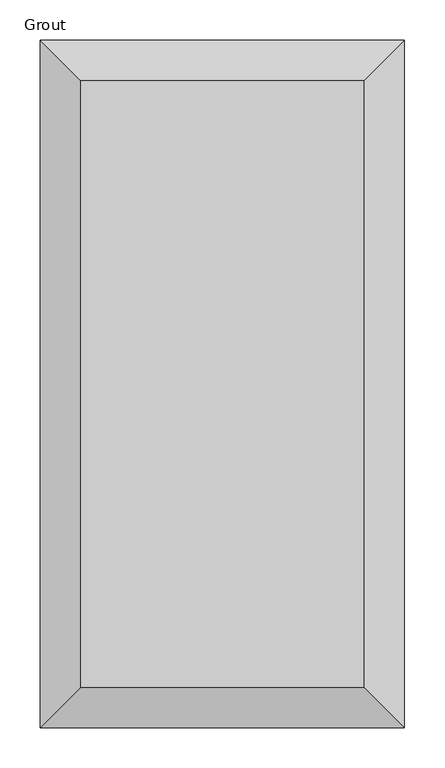
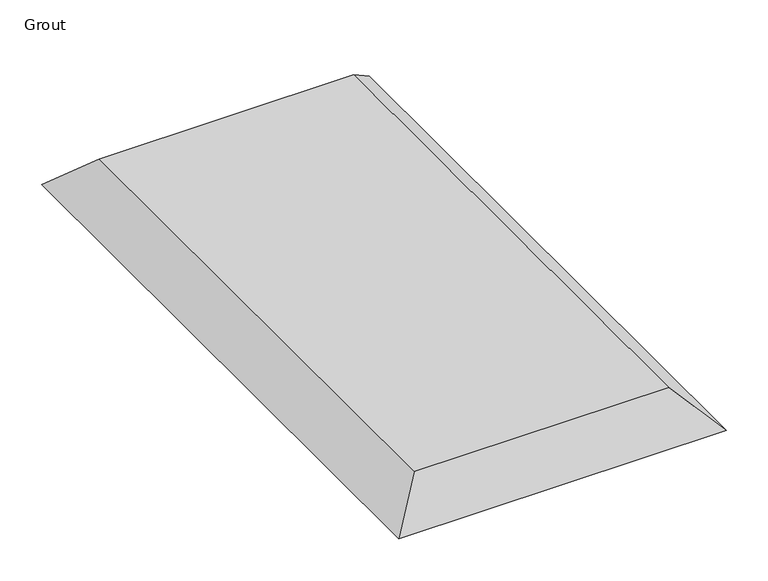
"""IFC4 building model written with IfcOpenShell, lengths in millimetres: proxy geometry, Grout : H_GM_AMM_Grouting_T50."""

from ifc_helpers import new_model, si_unit, origin, place, context, project, spatial, faceted_brep, source, transform, mapped, element, save


def grout_43c68623(model_context):
    return source(origin(), model_context, "Body", "Brep", [
        faceted_brep([(175.0, 375.0, 863.9720055), (-175.0, 375.0, 863.9720055), (-175.0, -375.0, 863.9720055), (175.0, -375.0, 863.9720055), (225.0, 425.0, 813.9720055), (225.0, -425.0, 813.9720055), (-225.0, -425.0, 813.9720055), (-225.0, 425.0, 813.9720055)], [[[0, 1, 2, 3]], [[4, 5, 6, 7]], [[4, 7, 1, 0]], [[7, 6, 2, 1]], [[6, 5, 3, 2]], [[5, 4, 0, 3]]]),
    ])


if __name__ == "__main__":
    model = new_model("IFC4")
    model_context = context("Model", 3, world=origin())
    ifc_project = project(units=[si_unit("LENGTHUNIT", "METRE", prefix="MILLI")], contexts=[model_context])
    site = spatial("IfcSite", under=ifc_project)
    building = spatial("IfcBuilding", under=site)
    placement = place(None, origin())
    grout_shape = grout_43c68623(model_context)
    element("IfcBuildingElementProxy", 1, Name="Grout : H_GM_AMM_Grouting_T50", ObjectType="Grout : H_GM_AMM_Grouting_T50", at=placement, inside=building, context=model_context, shape_type="MappedRepresentation", body=[
        mapped(grout_shape, transform((0.0, 0.0, 0.0), x_axis=(1.0, 0.0, 0.0), y_axis=(0.0, 1.0, 0.0), z_axis=(0.0, 0.0, 1.0))),
    ])
    save(model, "model.ifc")
